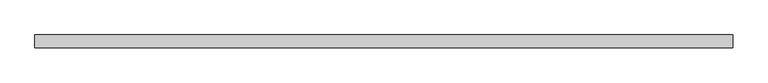
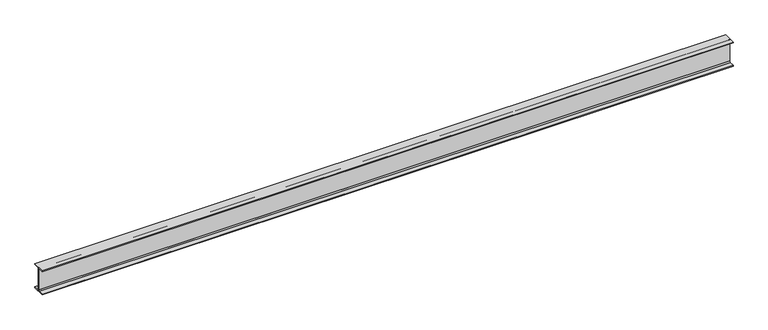
"""IFC4 building model written with IfcOpenShell, lengths in millimetres: beam geometry, 0912_Steel Framing_H-KSD3502 : H_SB_ASB_H-350x175x7x11."""

import ifcopenshell
import ifcopenshell.guid

model = None  # the IFC model being written
_history = None  # IfcOwnerHistory: only IFC2X3 demands one
_inside = {}  # id of a spatial element -> (the spatial element, [elements in it])
_under = {}  # id of a project, library or spatial element -> (it, [spatial elements below it])
_declared = {}  # id of a project -> (the project, [libraries it declares])
_typed = {}  # id of a type object -> (the type object, [elements of that type])
_made_of = {}  # id of a material, layer set ... -> (it, [elements and type objects made of it])


def new_model(schema):
    """Start an empty IFC model of exactly this schema.

    Asked for "IFC4X3", IfcOpenShell would pick the latest addendum, in which some entities
    have other attributes; the version numbers below select the first issue.
    IFC2X3 requires an IfcOwnerHistory on every rooted entity: one is made here for all.
    """
    global model, _history
    if schema == "IFC4X3":
        model = ifcopenshell.file(schema_version=(4, 3, 0, 0))
    else:
        model = ifcopenshell.file(schema=schema)
    _inside.clear()
    _under.clear()
    _declared.clear()
    _typed.clear()
    _made_of.clear()
    _history = None
    if model.schema == "IFC2X3":
        org = make("IfcOrganization", Name="unknown")
        user = make(
            "IfcPersonAndOrganization",
            ThePerson=make("IfcPerson", FamilyName="unknown"),
            TheOrganization=org,
        )
        app = make(
            "IfcApplication",
            ApplicationDeveloper=org,
            Version="unknown",
            ApplicationFullName="unknown",
            ApplicationIdentifier="unknown",
        )
        _history = make(
            "IfcOwnerHistory",
            OwningUser=user,
            OwningApplication=app,
            ChangeAction="ADDED",
            CreationDate=0,
        )
    return model


def make(cls, **values):
    """One entity of the class cls with the attributes given. An attribute that is None is left unset."""
    return model.create_entity(
        cls, **{name: value for name, value in values.items() if value is not None}
    )


def rooted(cls, **values):
    """An entity with a GlobalId (a new one), such as an element, a storey or a relation."""
    return make(cls, GlobalId=ifcopenshell.guid.new(), OwnerHistory=_history, **values)


def si_unit(unit_type, name, prefix=None):
    """IfcSIUnit, for example si_unit("LENGTHUNIT", "METRE", prefix="MILLI")."""
    return make("IfcSIUnit", UnitType=unit_type, Prefix=prefix, Name=name)


def assignment(units):
    """IfcUnitAssignment: the units of a project."""
    return None if units is None else make("IfcUnitAssignment", Units=units)


def point(xyz):
    """IfcCartesianPoint."""
    return None if xyz is None else make("IfcCartesianPoint", Coordinates=xyz)


def direction(xyz):
    """IfcDirection."""
    return None if xyz is None else make("IfcDirection", DirectionRatios=xyz)


def frame(location, z_axis=None, x_axis=None):
    """IfcAxis2Placement3D, a coordinate frame: its origin and axes. An axis left out is left unset."""
    return make(
        "IfcAxis2Placement3D",
        Location=point(location),
        Axis=direction(z_axis),
        RefDirection=direction(x_axis),
    )


def frame_2d(location, x_axis=None):
    """IfcAxis2Placement2D, a coordinate frame in the plane: its origin and x axis."""
    return make(
        "IfcAxis2Placement2D", Location=point(location), RefDirection=direction(x_axis)
    )


def origin():
    """The frame at (0, 0, 0) with its axes left unset."""
    return frame((0.0, 0.0, 0.0))


def place(relative_to, where):
    """IfcLocalPlacement: puts the frame where relative to a parent placement (None: the world)."""
    return make(
        "IfcLocalPlacement", PlacementRelTo=relative_to, RelativePlacement=where
    )


def context(
    kind, dimensions, precision=None, world=None, true_north=None, identifier=None
):
    """IfcGeometricRepresentationContext, for example the 3D "Model" context."""
    return make(
        "IfcGeometricRepresentationContext",
        ContextIdentifier=identifier,
        ContextType=kind,
        CoordinateSpaceDimension=dimensions,
        Precision=precision,
        WorldCoordinateSystem=world,
        TrueNorth=true_north,
    )


def project(units=None, contexts=None):
    """IfcProject with its units and contexts."""
    return rooted(
        "IfcProject",
        Name="project",
        RepresentationContexts=contexts,
        UnitsInContext=assignment(units),
    )


def spatial(cls, under=None, at=None, **own):
    """A site, building, storey or space (cls), placed at a placement, below another one or the project."""
    s = rooted(cls, ObjectPlacement=at, **own)
    if under is not None:
        _under.setdefault(under.id(), (under, []))[1].append(s)
    return s


def polyline(points):
    """IfcPolyline through the points."""
    return make("IfcPolyline", Points=[point(p) for p in points])


def circle_curve(where, radius):
    """IfcCircle in the frame where."""
    return make("IfcCircle", Position=where, Radius=radius)


def trimmed(basis, trim1, trim2, sense, master):
    """IfcTrimmedCurve: the piece of a basis curve between two trims."""
    return make(
        "IfcTrimmedCurve",
        BasisCurve=basis,
        Trim1=trim1,
        Trim2=trim2,
        SenseAgreement=sense,
        MasterRepresentation=master,
    )


def segment(curve, same_sense, transition):
    """IfcCompositeCurveSegment."""
    return make(
        "IfcCompositeCurveSegment",
        Transition=transition,
        SameSense=same_sense,
        ParentCurve=curve,
    )


def composite_curve(segments, self_intersect=None):
    """IfcCompositeCurve: segments joined end to end."""
    return make("IfcCompositeCurve", Segments=segments, SelfIntersect=self_intersect)


def outline(outer, holes=None, kind="AREA"):
    """IfcArbitraryClosedProfileDef: a profile drawn as a closed curve; with holes, ...WithVoids."""
    if holes is None:
        return make("IfcArbitraryClosedProfileDef", ProfileType=kind, OuterCurve=outer)
    return make(
        "IfcArbitraryProfileDefWithVoids",
        ProfileType=kind,
        OuterCurve=outer,
        InnerCurves=holes,
    )


def extrude(swept, where, along, depth):
    """IfcExtrudedAreaSolid: the profile swept, set in the frame where, extruded along a direction by depth."""
    return make(
        "IfcExtrudedAreaSolid",
        SweptArea=swept,
        Position=where,
        ExtrudedDirection=direction(along),
        Depth=depth,
    )


def shape(context_of_items, identifier, shape_type, items):
    """IfcShapeRepresentation: the items that make up one representation, for example the "Body"."""
    return make(
        "IfcShapeRepresentation",
        ContextOfItems=context_of_items,
        RepresentationIdentifier=identifier,
        RepresentationType=shape_type,
        Items=items,
    )


def source(mapping_origin, context_of_items, identifier, shape_type, items):
    """IfcRepresentationMap: a shape defined once, which mapped items show again and again."""
    return make(
        "IfcRepresentationMap",
        MappingOrigin=mapping_origin,
        MappedRepresentation=shape(context_of_items, identifier, shape_type, items),
    )


def transform(
    local_origin,
    x_axis=None,
    y_axis=None,
    z_axis=None,
    scale=None,
    scale2=None,
    scale3=None,
    uniform=True,
):
    """IfcCartesianTransformationOperator3D, or its non-uniform kind. x_axis, y_axis, z_axis: its Axis1, 2, 3."""
    if uniform:
        return make(
            "IfcCartesianTransformationOperator3D",
            Axis1=direction(x_axis),
            Axis2=direction(y_axis),
            LocalOrigin=point(local_origin),
            Scale=scale,
            Axis3=direction(z_axis),
        )
    return make(
        "IfcCartesianTransformationOperator3DnonUniform",
        Axis1=direction(x_axis),
        Axis2=direction(y_axis),
        LocalOrigin=point(local_origin),
        Scale=scale,
        Axis3=direction(z_axis),
        Scale2=scale2,
        Scale3=scale3,
    )


def mapped(mapping_source, mapping_target):
    """IfcMappedItem: shows the shape of a source again, moved by a transform."""
    return make(
        "IfcMappedItem", MappingSource=mapping_source, MappingTarget=mapping_target
    )


def made_of(thing, what):
    """Note that an element or type object is made of a material, layer set ...; save() writes the relation."""
    if what is not None:
        _made_of.setdefault(what.id(), (what, []))[1].append(thing)
    return thing


def element(
    cls,
    number,
    at=None,
    inside=None,
    cuts=None,
    type_object=None,
    material=None,
    context=None,
    identifier="Body",
    shape_type=None,
    held_by="IfcProductDefinitionShape",
    body=None,
    shapes=None,
    **own,
):
    """One element of the class cls, such as IfcWall. Its Tag is "e" and its number.

    at: its placement. inside: the storey or other place that contains it. cuts: it is an
    opening in that element (IfcRelVoidsElement). A single representation is given by context,
    identifier, shape_type and body (its items); several are given by shapes. held_by: the class
    of the entity that holds the representations. save() writes the other relations.
    """
    e = rooted(cls, Tag="e%d" % number, ObjectPlacement=at, **own)
    if body is not None:
        shapes = [shape(context, identifier, shape_type, body)]
    if shapes is not None:
        e.Representation = make(held_by, Representations=shapes)
    if inside is not None:
        _inside.setdefault(inside.id(), (inside, []))[1].append(e)
    if cuts is not None:
        rooted(
            "IfcRelVoidsElement", RelatingBuildingElement=cuts, RelatedOpeningElement=e
        )
    if type_object is not None:
        _typed.setdefault(type_object.id(), (type_object, []))[1].append(e)
    return made_of(e, material)


def aggregate(whole, parts):
    """IfcRelAggregates: a whole, such as a stair, and the parts it consists of."""
    return rooted("IfcRelAggregates", RelatingObject=whole, RelatedObjects=parts)


def save(model, path):
    """Write the relations noted so far, then the file.

    IfcRelAggregates (storeys below a building ...), IfcRelContainedInSpatialStructure (elements
    in a storey), IfcRelDefinesByType, IfcRelAssociatesMaterial and IfcRelDeclares: one each for
    every whole, place, type object, material and project.
    """
    for whole, parts in _under.values():
        aggregate(whole, parts)
    for where, things in _inside.values():
        rooted(
            "IfcRelContainedInSpatialStructure",
            RelatedElements=things,
            RelatingStructure=where,
        )
    for kind, things in _typed.values():
        rooted("IfcRelDefinesByType", RelatedObjects=things, RelatingType=kind)
    for what, things in _made_of.values():
        rooted("IfcRelAssociatesMaterial", RelatedObjects=things, RelatingMaterial=what)
    for by, libraries in _declared.values():
        rooted("IfcRelDeclares", RelatingContext=by, RelatedDefinitions=libraries)
    model.write(path)


def beam_f28858a7(model_context):
    return source(origin(), model_context, "Body", "SweptSolid", [
        extrude(outline(composite_curve([segment(polyline([(87.5, -164.0), (87.5, -175.0), (-87.5, -175.0), (-87.5, -164.0), (-17.5, -164.0)]), True, "CONTINUOUS"), segment(trimmed(circle_curve(frame_2d((-17.5, -150.0)), 14.0), [point((-17.5, -164.0))], [point((-3.5, -150.0))], True, "CARTESIAN"), True, "CONTINUOUS"), segment(polyline([(-3.5, -150.0), (-3.5, 150.0)]), True, "CONTINUOUS"), segment(trimmed(circle_curve(frame_2d((-17.5, 150.0)), 14.0), [point((-3.5, 150.0))], [point((-17.5, 164.0))], True, "CARTESIAN"), True, "CONTINUOUS"), segment(polyline([(-17.5, 164.0), (-87.5, 164.0), (-87.5, 175.0), (87.5, 175.0), (87.5, 164.0), (17.5, 164.0)]), True, "CONTINUOUS"), segment(trimmed(circle_curve(frame_2d((17.5, 150.0)), 14.0), [point((17.5, 164.0))], [point((3.5, 150.0))], True, "CARTESIAN"), True, "CONTINUOUS"), segment(polyline([(3.5, 150.0), (3.5, -150.0)]), True, "CONTINUOUS"), segment(trimmed(circle_curve(frame_2d((17.5, -150.0)), 14.0), [point((3.5, -150.0))], [point((17.5, -164.0))], True, "CARTESIAN"), True, "CONTINUOUS"), segment(polyline([(17.5, -164.0), (87.5, -164.0)]), True, "CONTINUOUS")], self_intersect=False)), frame((-4664.4729123, 0.0, 0.0), z_axis=(1.0, 0.0, 0.0), x_axis=(0.0, 1.0, 0.0)), (0.0, 0.0, 1.0), 9526.7729123),
    ])


if __name__ == "__main__":
    model = new_model("IFC4")
    model_context = context("Model", 3, world=origin())
    ifc_project = project(units=[si_unit("LENGTHUNIT", "METRE", prefix="MILLI")], contexts=[model_context])
    site = spatial("IfcSite", under=ifc_project)
    building = spatial("IfcBuilding", under=site)
    placement = place(None, origin())
    beam_shape = beam_f28858a7(model_context)
    element("IfcBeam", 1, ObjectType="0912_Steel Framing_H-KSD3502 : H_SB_ASB_H-350x175x7x11", at=placement, inside=building, context=model_context, shape_type="MappedRepresentation", body=[
        mapped(beam_shape, transform((0.0, 0.0, 0.0), x_axis=(1.0, 0.0, 0.0), y_axis=(0.0, 1.0, 0.0), z_axis=(0.0, 0.0, 1.0))),
    ])
    save(model, "model.ifc")

# Revit data of these elements
# Type "0912_Steel Framing_H-KSD3502 : H_SB_ASB_H-350x175x7x11"
#   H_WM Code_1 = "S01AA002-00001 | Main Steel Structure Fabrication Work | Shelter/Building | Medium Steel - Standard (90KG/M>Weight≥30KG/M) | Material: (   )"
#   H_WM Code_2 = "S03AA028-00001 | Main Steel Structure Erection Work | Shelter/Building | Medium Steel (90KG/M>Weight≥30KG/M) | Material: (   )"
#   H_WM Code_3 = "S01AA010-00001 | Main Steel Structure Fabrication Work | Shelter/Building | Steel Painting/Coating | for Non-Fireproofed Steel Surface, Surface Preparation, Primer, Second & Final Coat | Material: (   )"
#   H_Q'ty Cal Type Tag = "SB-Q2"
#   Width = 17.5 cm
#   Web Thickness = 0.7 cm
#   Web Fillet = 1.4 cm
#   Warping Constant = 282000.0 cm⁶
#   W = 0
#   Torsional Moment of Inertia = 19.4042 cm⁴
#   Section Area = 63.14 cm²
#   Plastic Modulus weak axis = 174.0 cm³
#   Plastic Modulus strong axis = 868.0 cm³
#   Perimeter = 1.36 m²/m
#   Nominal Weight = 49.60 kgf/m
#   Moment of Inertia weak axis = 984.00 cm⁴
#   Moment of Inertia strong axis = 13600.00 cm⁴
#   Height = 35.0 cm
#   Flange Thickness = 1.1 cm
#   Elastic Modulus weak axis = 112.0 cm³
#   Elastic Modulus strong axis = 775.0 cm³
#   Centroid Vertical = 17.5 cm
#   Centroid Horizontal = 8.75 cm
#   Ix = 136000000
#   Length [instance default] = 1.5240 m
#   Zx = 868000
#   b = 0.1750 m
#   h = 0.3500 m
#   r = 0.0140 m
#   s = 0.0070 m
#   t = 0.0110 m
#   A = 0.006314 m²
#   Structural Material [instance default] = Steel, 45-345
#   Assembly Code = ""
# Element 1 (IfcBeam, "0912_Steel Framing_H-KSD3502 : H_SB_ASB_H-350x175x7x11")
#   Structural Material = none
# Materials
#   "Steel, 45-345": class "Metal", colour RGB 189 187 185, transparency 0, Description = "Steel 345 MPa", Cost = 0
